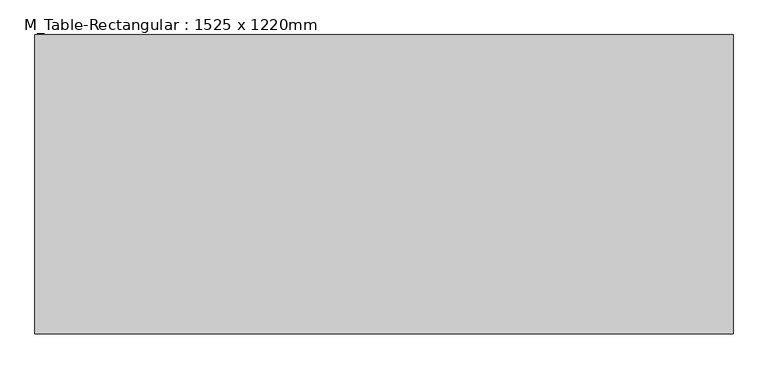
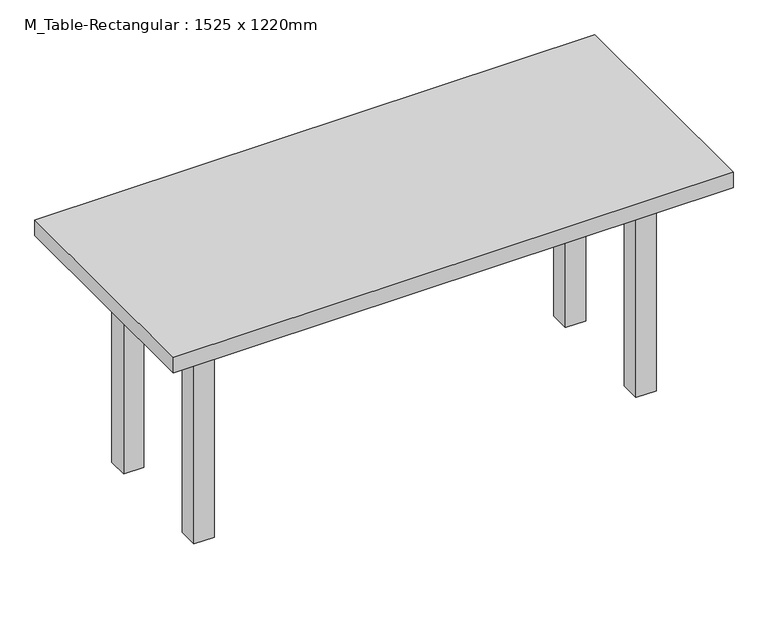
"""IFC4 building model written with IfcOpenShell, lengths in millimetres: furniture geometry, M_Table-Rectangular : 1525 x 1220mm."""

from ifc_helpers import new_model, si_unit, frame, origin, origin_with_axes, place, context, project, spatial, polyline, outline, extrude, source, transform, mapped, element, save


def m_table_rectangular_1525_x_1220mm_22d60bad(model_context):
    return source(origin(), model_context, "Body", "SweptSolid", [
        extrude(outline(polyline([(659.1, 184.5), (659.1, 159.1), (-659.1, 159.1), (-659.1, 184.5), (659.1, 184.5)])), frame((0.0, 0.0, 609.6), z_axis=(0.0, 0.0, 1.0), x_axis=(1.0, 0.0, 0.0)), (0.0, 0.0, 1.0), 101.6),
        extrude(outline(polyline([(659.1, -184.5), (-659.1, -184.5), (-659.1, -159.1), (659.1, -159.1), (659.1, -184.5)])), frame((0.0, 0.0, 609.6), z_axis=(0.0, 0.0, 1.0), x_axis=(1.0, 0.0, 0.0)), (0.0, 0.0, 1.0), 101.6),
        extrude(outline(polyline([(-671.8, -159.1), (-697.2, -159.1), (-697.2, 159.1), (-671.8, 159.1), (-671.8, -159.1)])), frame((0.0, 0.0, 609.6), z_axis=(0.0, 0.0, 1.0), x_axis=(1.0, 0.0, 0.0)), (0.0, 0.0, 1.0), 101.6),
        extrude(outline(polyline([(671.8, -159.1), (671.8, 159.1), (697.2, 159.1), (697.2, -159.1), (671.8, -159.1)])), frame((0.0, 0.0, 609.6), z_axis=(0.0, 0.0, 1.0), x_axis=(1.0, 0.0, 0.0)), (0.0, 0.0, 1.0), 101.6),
        extrude(outline(polyline([(875.0, 375.0), (875.0, -375.0), (-875.0, -375.0), (-875.0, 375.0), (875.0, 375.0)])), frame((0.0, 0.0, 711.2), z_axis=(0.0, 0.0, 1.0), x_axis=(1.0, 0.0, 0.0)), (0.0, 0.0, 1.0), 50.8),
        extrude(outline(polyline([(-659.1, 222.6), (-659.1, 159.1), (-722.6, 159.1), (-722.6, 222.6), (-659.1, 222.6)])), origin_with_axes(), (0.0, 0.0, 1.0), 711.2),
        extrude(outline(polyline([(659.1, 222.6), (722.6, 222.6), (722.6, 159.1), (659.1, 159.1), (659.1, 222.6)])), origin_with_axes(), (0.0, 0.0, 1.0), 711.2),
        extrude(outline(polyline([(-659.1, -222.6), (-722.6, -222.6), (-722.6, -159.1), (-659.1, -159.1), (-659.1, -222.6)])), origin_with_axes(), (0.0, 0.0, 1.0), 711.2),
        extrude(outline(polyline([(659.1, -222.6), (659.1, -159.1), (722.6, -159.1), (722.6, -222.6), (659.1, -222.6)])), origin_with_axes(), (0.0, 0.0, 1.0), 711.2),
    ])


if __name__ == "__main__":
    model = new_model("IFC4")
    model_context = context("Model", 3, world=origin())
    ifc_project = project(units=[si_unit("LENGTHUNIT", "METRE", prefix="MILLI")], contexts=[model_context])
    site = spatial("IfcSite", under=ifc_project)
    building = spatial("IfcBuilding", under=site)
    placement = place(None, origin())
    m_table_rectangular_1525_x_1220mm_shape = m_table_rectangular_1525_x_1220mm_22d60bad(model_context)
    element("IfcFurniture", 1, ObjectType="M_Table-Rectangular : 1525 x 1220mm", at=placement, inside=building, context=model_context, shape_type="MappedRepresentation", body=[
        mapped(m_table_rectangular_1525_x_1220mm_shape, transform((0.0, 0.0, 0.0), x_axis=(1.0, 0.0, 0.0), y_axis=(0.0, 1.0, 0.0), z_axis=(0.0, 0.0, 1.0))),
    ])
    save(model, "model.ifc")

# Revit data of these elements
# Type "M_Table-Rectangular : 1525 x 1220mm"
#   Height = 0.762 m
#   Length = 1.75 m
#   Width = 0.75 m
#   Base Material = Birch
#   Top Material = Birch
# Element 1 (IfcFurniture, "M_Table-Rectangular : 1525 x 1220mm")
#   Materials on its faces: "Birch"
# Materials
#   "Birch": class "Wood", colour RGB 224 178 126, transparency 0, Description = "Betula Alleghaniensis", Cost = 0
